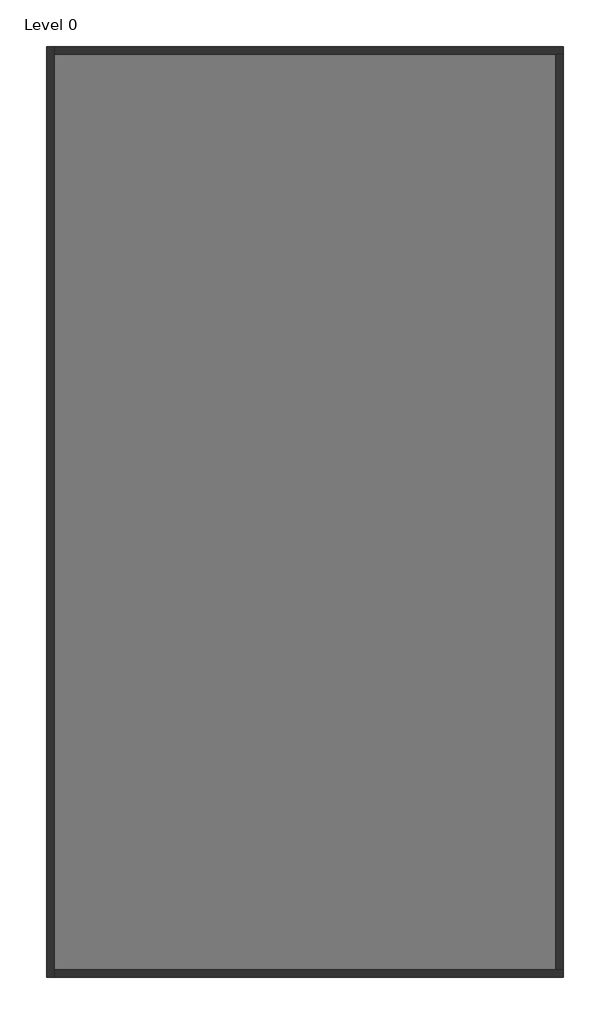
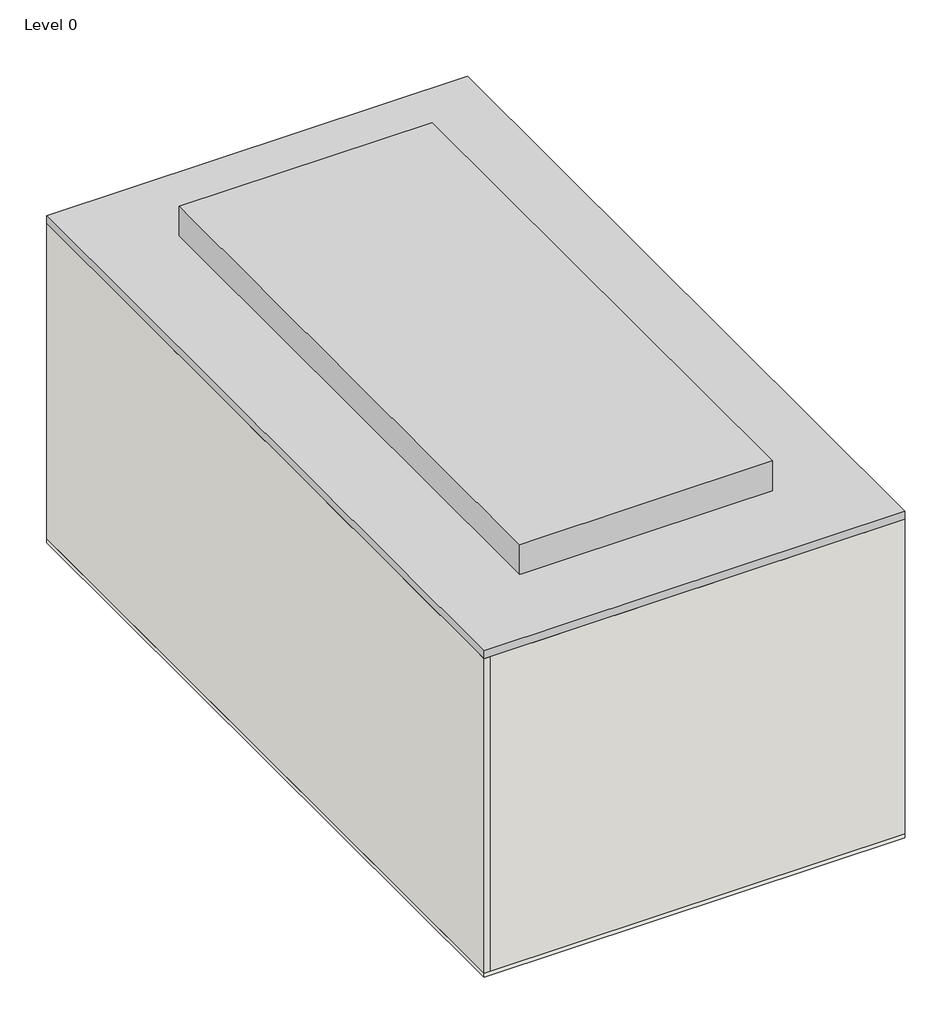
# One storey: 4 walls, 1 proxy, 1 slab.
"""IFC4 building model written with IfcOpenShell, lengths in millimetres."""

from ifc_helpers import new_model, si_unit, frame, origin, origin_with_axes, place, context, project, spatial, polyline, outline, extrude, faceted_brep, element, save

model = new_model("IFC4")

# Units and contexts
model_context = context("Model", 3, world=origin())
ifc_project = project(units=[si_unit("LENGTHUNIT", "METRE", prefix="MILLI")], contexts=[model_context])

# Site, building, storey
site = spatial("IfcSite", under=ifc_project)
building = spatial("IfcBuilding", under=site)
storey = spatial("IfcBuildingStorey", under=building, Name="Level 0", Elevation=100.0)

# Proxy
placement = place(None, origin())
element("IfcBuildingElementProxy", 1, Name="LowUrbanDensityBuilding : LowUrbanDensityBuilding", ObjectType="LowUrbanDensityBuilding : LowUrbanDensityBuilding", at=placement, inside=storey, context=model_context, shape_type="SweptSolid", body=[
    extrude(outline(polyline([(7325.2659446, 3676.2074539), (7325.2659446, -14323.7925461), (-2674.7340554, -14323.7925461), (-2674.7340554, 3676.2074539), (7325.2659446, 3676.2074539)])), origin_with_axes(), (0.0, 0.0, 1.0), 8200.0),
    extrude(outline(polyline([(5325.2659446, 1676.2074539), (5325.2659446, -12323.7925461), (-674.7340554, -12323.7925461), (-674.7340554, 1676.2074539), (5325.2659446, 1676.2074539)])), frame((0.0, 0.0, 8200.0), z_axis=(0.0, 0.0, 1.0), x_axis=(1.0, 0.0, 0.0)), (0.0, 0.0, 1.0), 749.8),
])

# Slab
element("IfcSlab", 2, ObjectType="Floor-Concrete_100Con", at=placement, inside=storey, context=model_context, shape_type="SweptSolid", body=[
    extrude(outline(polyline([(7325.2659446, 3676.2074539), (7325.2659446, -14323.7925461), (-2674.7340554, -14323.7925461), (-2674.7340554, 3676.2074539), (7325.2659446, 3676.2074539)])), origin_with_axes(), (0.0, 0.0, 1.0), 100.0),
])

# Walls
element("IfcWall", 3, ObjectType="Wall-Ext_25Rdr-100Blk-19P", at=placement, inside=storey, context=model_context, shape_type="Brep", body=[
    faceted_brep([(-2674.7340554, 3676.2074539, 100.0), (-2674.7340554, -14323.7925461, 100.0), (-2674.7340554, -14323.7925461, 8000.0), (-2674.7340554, 3676.2074539, 8000.0), (-2530.4340554, 3676.2074539, 100.0), (-2530.4340554, 3676.2074539, 8000.0), (-2530.4340554, 3531.9074539, 8000.0), (-2530.4340554, -14179.4925461, 8000.0), (-2530.4340554, -14323.7925461, 8000.0), (-2530.4340554, -14323.7925461, 100.0), (-2530.4340554, -14179.4925461, 100.0), (-2530.4340554, 3531.9074539, 100.0)], [[[0, 1, 2, 3]], [[4, 5, 6, 7, 8, 9, 10, 11]], [[1, 0, 4, 11, 10, 9]], [[3, 2, 8, 7, 6, 5]], [[2, 1, 9, 8]], [[0, 3, 5, 4]]]),
])
element("IfcWall", 4, ObjectType="Wall-Ext_25Rdr-100Blk-19P", at=placement, inside=storey, context=model_context, shape_type="Brep", body=[
    faceted_brep([(-2530.4340554, -14323.7925461, 100.0), (7325.2659446, -14323.7925461, 100.0), (7325.2659446, -14323.7925461, 8000.0), (-2530.4340554, -14323.7925461, 8000.0), (-2530.4340554, -14179.4925461, 100.0), (-2530.4340554, -14179.4925461, 8000.0), (7180.9659446, -14179.4925461, 8000.0), (7325.2659446, -14179.4925461, 8000.0), (7325.2659446, -14179.4925461, 100.0), (7180.9659446, -14179.4925461, 100.0)], [[[0, 1, 2, 3]], [[4, 5, 6, 7, 8, 9]], [[1, 0, 4, 9, 8]], [[3, 2, 7, 6, 5]], [[0, 3, 5, 4]], [[2, 1, 8, 7]]]),
])
element("IfcWall", 5, ObjectType="Wall-Ext_25Rdr-100Blk-19P", at=placement, inside=storey, context=model_context, shape_type="Brep", body=[
    faceted_brep([(7325.2659446, 3676.2074539, 100.0), (-2530.4340554, 3676.2074539, 100.0), (-2530.4340554, 3676.2074539, 8000.0), (7325.2659446, 3676.2074539, 8000.0), (7325.2659446, 3531.9074539, 100.0), (7325.2659446, 3531.9074539, 8000.0), (7180.9659446, 3531.9074539, 8000.0), (-2530.4340554, 3531.9074539, 8000.0), (-2530.4340554, 3531.9074539, 100.0), (7180.9659446, 3531.9074539, 100.0)], [[[0, 1, 2, 3]], [[4, 5, 6, 7, 8, 9]], [[1, 0, 4, 9, 8]], [[3, 2, 7, 6, 5]], [[2, 1, 8, 7]], [[0, 3, 5, 4]]]),
])
element("IfcWall", 6, ObjectType="Wall-Ext_25Rdr-100Blk-19P", at=placement, inside=storey, context=model_context, shape_type="SweptSolid", body=[
    extrude(outline(polyline([(7325.2659446, 3531.9074539), (7325.2659446, -14179.4925461), (7180.9659446, -14179.4925461), (7180.9659446, 3531.9074539), (7325.2659446, 3531.9074539)])), frame((0.0, 0.0, 100.0), z_axis=(0.0, 0.0, 1.0), x_axis=(1.0, 0.0, 0.0)), (0.0, 0.0, 1.0), 7900.0),
])

save(model, "model.ifc")

# Revit data of these elements
# Project information
#   Project Issue Date = "Issue Date"
#   Project Status = "Project Status"
#   Client Name = "Owner"
#   Project Address = "Enter address here"
#   Project Name = "Project Name"
#   Project Number = "Project Number"
# Type "Floor-Concrete_100Con"
#   Keynote = "E60/130"
#   Function = 0
#   Layers, outside or top first: 100 mm "Concrete" (function 1)
# Type "Wall-Ext_25Rdr-100Blk-19P"
#   Keynote = "F10"
#   Layers, outside or top first: 25.3 mm "Render, Beige, Smooth" (function 5); 100 mm "Concrete Masonry Units _Low Density" (function 1); 19 mm "Plaster" (function 5)
# Element 1 (IfcBuildingElementProxy, "LowUrbanDensityBuilding : LowUrbanDensityBuilding")
#   Phase Created = New Construction
#   Materials on its faces: "Default Form"
# Element 2 (IfcSlab, "Floor-Concrete_100Con")
#   Height Offset From Level = 0 mm
#   Phase Created = New Construction
#   Materials on its faces: "Concrete"
# Element 3 (IfcWall, "Wall-Ext_25Rdr-100Blk-19P")
#   Top Offset = 0 mm
#   Base Offset = 0 mm
#   wall height = 7900 mm
#   Phase Created = New Construction
#   Base Constraint = Level 0
#   Top Constraint = Level 2
#   Materials on its faces: "Render, Beige, Smooth", "Default Wall", "Plaster"
# Elements 4, 5, 6 (IfcWall, "Wall-Ext_25Rdr-100Blk-19P")
#   Top Offset = 0 mm
#   Base Offset = 0 mm
#   wall height = 7900 mm
#   Phase Created = New Construction
#   Base Constraint = Level 0
#   Top Constraint = Level 2
#   Materials on its faces: "Default Wall", "Render, Beige, Smooth", "Plaster"
# Materials
#   "Concrete": class "Concrete", colour RGB 120 120 120, transparency 0, Description = "Portland Cement Concrete", Cost = 0
#   "Render, Beige, Smooth": class "Generic", colour RGB 213 198 180, transparency 0, Description = "physical material", Cost = 0
#   "Concrete Masonry Units _Low Density": class "Masonry", colour RGB 181 181 181, transparency 0, Description = "Concrete masonry units", Cost = 0
#   "Plaster": class "Generic", colour RGB 249 249 249, transparency 0, Description = "Plaster", Cost = 0
#   "Default Form": class "Generic", colour RGB 185 189 196, transparency 0.5, Cost = 0
#   "Default Wall": class "Miscellaneous", colour RGB 128 128 128, transparency 0, Comments = "Rendering appearance not upgraded Rendering appearance not upgraded ", Cost = 0
